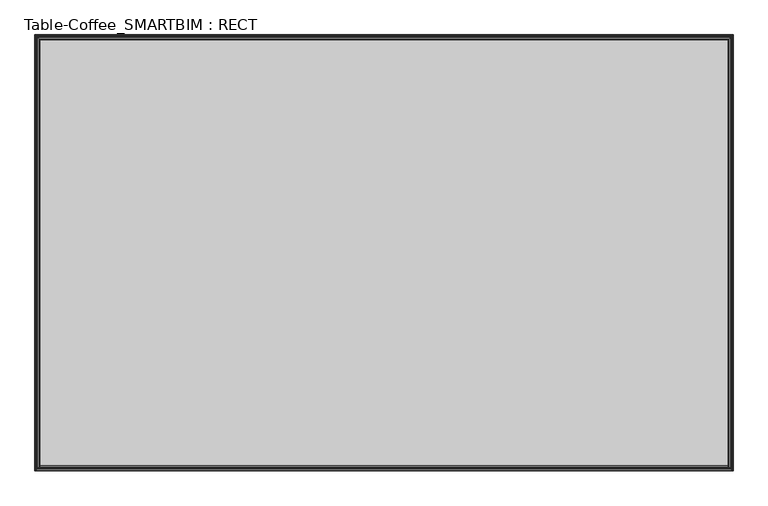
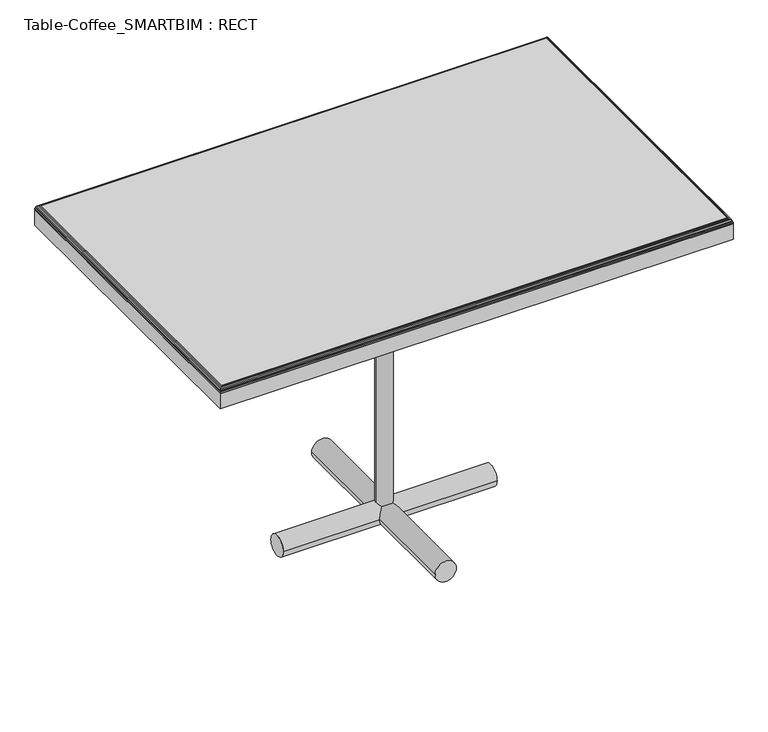
"""IFC4 building model written with IfcOpenShell, lengths in millimetres: furniture geometry, Table-Coffee_SMARTBIM : RECT."""

from ifc_helpers import new_model, si_unit, point, frame, frame_2d, origin, origin_2d, place, context, project, spatial, polyline, circle_curve, ellipse_curve, trimmed, segment, composite_curve, outline, extrude, source, transform, mapped, element, save
from ifc_brep_helpers import plane_surface, cylinder_surface, advanced_brep


def table_coffee_smartbim_rect_06f34b69(model_context):
    return source(origin(), model_context, "Body", "SolidModel", [
        extrude(outline(composite_curve([segment(trimmed(circle_curve(frame_2d((0.0, 25.4)), 25.4), [point((-25.4, 25.4))], [point((25.4, 25.4))], False, "CARTESIAN"), True, "CONTINUOUS"), segment(trimmed(circle_curve(frame_2d((0.0, 25.4)), 25.4), [point((25.4, 25.4))], [point((-25.4, 25.4))], False, "CARTESIAN"), True, "CONTINUOUS")], self_intersect=False)), frame((-254.0, 0.0, 0.0), z_axis=(1.0, 0.0, 0.0), x_axis=(0.0, 1.0, 0.0)), (0.0, 0.0, 1.0), 508.0),
        extrude(outline(composite_curve([segment(trimmed(circle_curve(frame_2d((25.4, 0.0)), 25.4), [point((25.4, -25.4))], [point((25.4, 25.4))], False, "CARTESIAN"), True, "CONTINUOUS"), segment(trimmed(circle_curve(frame_2d((25.4, 0.0)), 25.4), [point((25.4, 25.4))], [point((25.4, -25.4))], False, "CARTESIAN"), True, "CONTINUOUS")], self_intersect=False)), frame((0.0, -254.0, 0.0), z_axis=(0.0, 1.0, 0.0), x_axis=(0.0, 0.0, 1.0)), (0.0, 0.0, 1.0), 508.0),
        extrude(outline(polyline([(609.6, -381.0), (-609.6, -381.0), (-609.6, 381.0), (609.6, 381.0), (609.6, -381.0)])), frame((0.0, 0.0, 723.9), z_axis=(0.0, 0.0, 1.0), x_axis=(1.0, 0.0, 0.0)), (0.0, 0.0, 1.0), 38.1),
        advanced_brep(
        [(-600.1998654, 371.5998654, 774.7), (-600.1998654, -371.5998654, 774.7), (600.1998654, -371.5998654, 774.7), (600.1998654, 371.5998654, 774.7), (609.6, -381.0, 762.0), (-609.6, -381.0, 762.0), (-609.6, 381.0, 762.0), (609.6, 381.0, 762.0), (609.6, -381.0, 765.2998654), (-609.6, -381.0, 765.2998654), (-609.6, 381.0, 765.2998654), (609.6, 381.0, 765.2998654), (-609.2372483, -380.6372483, 767.8860287), (-609.2372483, 380.6372483, 767.8860287), (-602.3616212, -373.7616212, 774.4480533), (-602.3616212, 373.7616212, 774.4480533), (-604.3639185, 375.7639185, 773.7273912), (-604.3639185, -375.7639185, 773.7273912), (-606.4885738, 377.8885738, 772.2866155), (-606.4885738, -377.8885738, 772.2866155), (-608.5102962, 379.9102962, 769.692959), (-608.5102962, -379.9102962, 769.692959), (609.2372483, 380.6372483, 767.8860287), (602.3616212, 373.7616212, 774.4480533), (604.3639185, 375.7639185, 773.7273912), (606.4885738, 377.8885738, 772.2866155), (608.5102962, 379.9102962, 769.692959), (609.2372483, -380.6372483, 767.8860287), (602.3616212, -373.7616212, 774.4480533), (604.3639185, -375.7639185, 773.7273912), (606.4885738, -377.8885738, 772.2866155), (608.5102962, -379.9102962, 769.692959)],
        [
            (0, 1),
            (1, 2),
            (2, 3),
            (3, 0),
            (4, 5),
            (5, 6),
            (6, 7),
            (7, 4),
            (4, 8),
            (8, 9),
            (9, 5),
            (9, 10),
            (10, 6),
            (10, 11),
            (11, 7),
            (11, 8),
            (9, 12, ellipse_curve(frame((-600.1998654, -371.5998654, 765.2998654), z_axis=(-0.7071067811865475, 0.7071067811865475, 0.0), x_axis=(0.7071067811865474, 0.7071067811865476, 0.0)), 13.2937978, 9.4001346)),
            (12, 13),
            (13, 10, ellipse_curve(frame((-600.1998654, 371.5998654, 765.2998654), z_axis=(-0.7071067811865475, -0.7071067811865475, 0.0), x_axis=(-0.7071067811865474, 0.7071067811865476, 0.0)), 13.2937978, 9.4001346)),
            (14, 1, ellipse_curve(frame((-600.1998654, -371.5998654, 765.2998654), z_axis=(-0.7071067811865475, 0.7071067811865475, 0.0), x_axis=(0.7071067811865474, 0.7071067811865476, 0.0)), 13.2937978, 9.4001346)),
            (0, 15, ellipse_curve(frame((-600.1998654, 371.5998654, 765.2998654), z_axis=(-0.7071067811865475, -0.7071067811865475, 0.0), x_axis=(-0.7071067811865474, 0.7071067811865476, 0.0)), 13.2937978, 9.4001346)),
            (15, 14),
            (15, 16, ellipse_curve(frame((-600.1998654, 371.5998654, 765.2998654), z_axis=(-0.7071067811865475, -0.7071067811865475, 0.0), x_axis=(-0.7071067811865474, 0.7071067811865476, 0.0)), 13.2937978, 9.4001346)),
            (16, 17),
            (17, 14, ellipse_curve(frame((-600.1998654, -371.5998654, 765.2998654), z_axis=(-0.7071067811865475, 0.7071067811865475, 0.0), x_axis=(0.7071067811865474, 0.7071067811865476, 0.0)), 13.2937978, 9.4001346)),
            (16, 18, ellipse_curve(frame((-600.1998654, 371.5998654, 765.2998654), z_axis=(-0.7071067811865475, -0.7071067811865475, 0.0), x_axis=(-0.7071067811865474, 0.7071067811865476, 0.0)), 13.2937978, 9.4001346)),
            (18, 19),
            (19, 17, ellipse_curve(frame((-600.1998654, -371.5998654, 765.2998654), z_axis=(-0.7071067811865475, 0.7071067811865475, 0.0), x_axis=(0.7071067811865474, 0.7071067811865476, 0.0)), 13.2937978, 9.4001346)),
            (18, 20, ellipse_curve(frame((-600.1998654, 371.5998654, 765.2998654), z_axis=(-0.7071067811865475, -0.7071067811865475, 0.0), x_axis=(-0.7071067811865474, 0.7071067811865476, 0.0)), 13.2937978, 9.4001346)),
            (20, 21),
            (21, 19, ellipse_curve(frame((-600.1998654, -371.5998654, 765.2998654), z_axis=(-0.7071067811865475, 0.7071067811865475, 0.0), x_axis=(0.7071067811865474, 0.7071067811865476, 0.0)), 13.2937978, 9.4001346)),
            (12, 21, ellipse_curve(frame((-600.1998654, -371.5998654, 765.2998654), z_axis=(-0.7071067811865475, 0.7071067811865475, 0.0), x_axis=(0.7071067811865474, 0.7071067811865476, 0.0)), 13.2937978, 9.4001346)),
            (20, 13, ellipse_curve(frame((-600.1998654, 371.5998654, 765.2998654), z_axis=(-0.7071067811865475, -0.7071067811865475, 0.0), x_axis=(-0.7071067811865474, 0.7071067811865476, 0.0)), 13.2937978, 9.4001346)),
            (13, 22),
            (22, 11, ellipse_curve(frame((600.1998654, 371.5998654, 765.2998654), z_axis=(-0.7071067811865475, 0.7071067811865475, 0.0), x_axis=(0.7071067811865476, 0.7071067811865474, 0.0)), 13.2937978, 9.4001346)),
            (3, 23, ellipse_curve(frame((600.1998654, 371.5998654, 765.2998654), z_axis=(-0.7071067811865475, 0.7071067811865475, 0.0), x_axis=(0.7071067811865476, 0.7071067811865474, 0.0)), 13.2937978, 9.4001346)),
            (23, 15),
            (23, 24, ellipse_curve(frame((600.1998654, 371.5998654, 765.2998654), z_axis=(-0.7071067811865475, 0.7071067811865475, 0.0), x_axis=(0.7071067811865476, 0.7071067811865474, 0.0)), 13.2937978, 9.4001346)),
            (24, 16),
            (24, 25, ellipse_curve(frame((600.1998654, 371.5998654, 765.2998654), z_axis=(-0.7071067811865475, 0.7071067811865475, 0.0), x_axis=(0.7071067811865476, 0.7071067811865474, 0.0)), 13.2937978, 9.4001346)),
            (25, 18),
            (25, 26, ellipse_curve(frame((600.1998654, 371.5998654, 765.2998654), z_axis=(-0.7071067811865475, 0.7071067811865475, 0.0), x_axis=(0.7071067811865476, 0.7071067811865474, 0.0)), 13.2937978, 9.4001346)),
            (26, 20),
            (26, 22, ellipse_curve(frame((600.1998654, 371.5998654, 765.2998654), z_axis=(-0.7071067811865475, 0.7071067811865475, 0.0), x_axis=(0.7071067811865476, 0.7071067811865474, 0.0)), 13.2937978, 9.4001346)),
            (22, 27),
            (27, 8, ellipse_curve(frame((600.1998654, -371.5998654, 765.2998654), z_axis=(0.7071067811865475, 0.7071067811865475, 0.0), x_axis=(0.7071067811865474, -0.7071067811865476, 0.0)), 13.2937978, 9.4001346)),
            (2, 28, ellipse_curve(frame((600.1998654, -371.5998654, 765.2998654), z_axis=(0.7071067811865475, 0.7071067811865475, 0.0), x_axis=(0.7071067811865474, -0.7071067811865476, 0.0)), 13.2937978, 9.4001346)),
            (28, 23),
            (28, 29, ellipse_curve(frame((600.1998654, -371.5998654, 765.2998654), z_axis=(0.7071067811865475, 0.7071067811865475, 0.0), x_axis=(0.7071067811865474, -0.7071067811865476, 0.0)), 13.2937978, 9.4001346)),
            (29, 24),
            (29, 30, ellipse_curve(frame((600.1998654, -371.5998654, 765.2998654), z_axis=(0.7071067811865475, 0.7071067811865475, 0.0), x_axis=(0.7071067811865474, -0.7071067811865476, 0.0)), 13.2937978, 9.4001346)),
            (30, 25),
            (30, 31, ellipse_curve(frame((600.1998654, -371.5998654, 765.2998654), z_axis=(0.7071067811865475, 0.7071067811865475, 0.0), x_axis=(0.7071067811865474, -0.7071067811865476, 0.0)), 13.2937978, 9.4001346)),
            (31, 26),
            (31, 27, ellipse_curve(frame((600.1998654, -371.5998654, 765.2998654), z_axis=(0.7071067811865475, 0.7071067811865475, 0.0), x_axis=(0.7071067811865474, -0.7071067811865476, 0.0)), 13.2937978, 9.4001346)),
            (27, 12),
            (14, 28),
            (17, 29),
            (19, 30),
            (21, 31),
        ],
        [
            plane_surface(frame((-609.6, -381.0, 774.7), z_axis=(0.0, 0.0, 1.0), x_axis=(-1.0, 0.0, 0.0))),
            plane_surface(frame((-609.6, -381.0, 762.0), z_axis=(0.0, 0.0, -1.0), x_axis=(1.0, 0.0, 0.0))),
            plane_surface(frame((609.6, -381.0, 774.7), z_axis=(0.0, -1.0, 0.0), x_axis=(0.0, 0.0, -1.0))),
            plane_surface(frame((-609.6, -381.0, 774.7), z_axis=(-1.0, 0.0, 0.0), x_axis=(0.0, 0.0, -1.0))),
            plane_surface(frame((-609.6, 381.0, 774.7), z_axis=(0.0, 1.0, 0.0), x_axis=(0.0, 0.0, -1.0))),
            plane_surface(frame((609.6, 381.0, 774.7), z_axis=(1.0, 0.0, 0.0), x_axis=(0.0, 0.0, -1.0))),
            cylinder_surface(frame((-600.1998654, -381.0, 765.2998654), z_axis=(0.0, 1.0, 0.0), x_axis=(1.0, 0.0, 0.0)), 9.4001346),
            cylinder_surface(frame((-609.6, 371.5998654, 765.2998654), z_axis=(1.0, 0.0, 0.0), x_axis=(0.0, -1.0, 0.0)), 9.4001346),
            cylinder_surface(frame((600.1998654, 381.0, 765.2998654), z_axis=(0.0, -1.0, 0.0), x_axis=(-1.0, 0.0, 0.0)), 9.4001346),
            cylinder_surface(frame((609.6, -371.5998654, 765.2998654), z_axis=(-1.0, 0.0, 0.0), x_axis=(0.0, 1.0, 0.0)), 9.4001346),
        ],
        [
            (0, [[1, 2, 3, 4]]),
            (1, [[5, 6, 7, 8]]),
            (2, [[9, 10, 11, -5]]),
            (3, [[-11, 12, 13, -6]]),
            (4, [[-13, 14, 15, -7]]),
            (5, [[-15, 16, -9, -8]]),
            (6, [[-12, 17, 18, 19]]),
            (6, [[20, -1, 21, 22]]),
            (6, [[23, 24, 25, -22]]),
            (6, [[26, 27, 28, -24]]),
            (6, [[29, 30, 31, -27]]),
            (6, [[32, -30, 33, -18]]),
            (7, [[34, 35, -14, -19]]),
            (7, [[-4, 36, 37, -21]]),
            (7, [[-37, 38, 39, -23]]),
            (7, [[-39, 40, 41, -26]]),
            (7, [[-41, 42, 43, -29]]),
            (7, [[-43, 44, -34, -33]]),
            (8, [[45, 46, -16, -35]]),
            (8, [[-3, 47, 48, -36]]),
            (8, [[-48, 49, 50, -38]]),
            (8, [[-50, 51, 52, -40]]),
            (8, [[-52, 53, 54, -42]]),
            (8, [[-54, 55, -45, -44]]),
            (9, [[-10, -46, 56, -17]]),
            (9, [[57, -47, -2, -20]]),
            (9, [[58, -49, -57, -25]]),
            (9, [[59, -51, -58, -28]]),
            (9, [[60, -53, -59, -31]]),
            (9, [[-56, -55, -60, -32]]),
        ],
    ),
        extrude(outline(polyline([(76.2, -76.2), (-76.2, -76.2), (-76.2, 76.2), (76.2, 76.2), (76.2, -76.2)])), frame((0.0, 0.0, 755.65), z_axis=(0.0, 0.0, 1.0), x_axis=(1.0, 0.0, 0.0)), (0.0, 0.0, 1.0), 6.35),
        extrude(outline(composite_curve([segment(trimmed(circle_curve(origin_2d(), 19.05), [point((-19.05, 0.0))], [point((19.05, 0.0))], False, "CARTESIAN"), True, "CONTINUOUS"), segment(trimmed(circle_curve(origin_2d(), 19.05), [point((19.05, 0.0))], [point((-19.05, 0.0))], False, "CARTESIAN"), True, "CONTINUOUS")], self_intersect=False)), frame((0.0, 0.0, 24.2070278), z_axis=(0.0, 0.0, 1.0), x_axis=(1.0, 0.0, 0.0)), (0.0, 0.0, 1.0), 731.4429722),
    ])


if __name__ == "__main__":
    model = new_model("IFC4")
    model_context = context("Model", 3, world=origin())
    ifc_project = project(units=[si_unit("LENGTHUNIT", "METRE", prefix="MILLI")], contexts=[model_context])
    site = spatial("IfcSite", under=ifc_project)
    building = spatial("IfcBuilding", under=site)
    placement = place(None, origin())
    table_coffee_smartbim_rect_shape = table_coffee_smartbim_rect_06f34b69(model_context)
    element("IfcFurniture", 1, ObjectType="Table-Coffee_SMARTBIM : RECT", at=placement, inside=building, context=model_context, shape_type="MappedRepresentation", body=[
        mapped(table_coffee_smartbim_rect_shape, transform((0.0, 0.0, 0.0), x_axis=(1.0, 0.0, 0.0), y_axis=(0.0, 1.0, 0.0), z_axis=(0.0, 0.0, 1.0))),
    ])
    save(model, "model.ifc")

# Revit data of these elements
# Type "Table-Coffee_SMARTBIM : RECT"
#   Subcategory = "Table\r\n"
#   SmartBIM Object Created By = "SMARTBIM, LLC"
#   Manufacturer = "SMARTBIM"
#   Assembly Code = "E2020200"
#   95 CSI = "12500"
#   04 CSI = "12 50 00"
#   table cloth = 0' - 1 1/2"
#   Width = 4' - 0"
#   SmartBIM Object Version = 3
#   Height = 2' - 6"
#   Depth = 2' - 6"
#   Default Elevation = 4' - 0"
#   white cloth_parameter = WOOD-OAKFIRE
#   Table Unit = MET
#   Glide = none
#   Glass = none
# Element 1 (IfcFurniture, "Table-Coffee_SMARTBIM : RECT")
#   Materials on its faces: "WOOD-OAKFIRE", "MET"
# Materials
#   "WOOD-OAKFIRE": class "Wood", colour RGB 198 202 183, transparency 0, Description = "Generic wood", Cost = 0
#   "MET": class "Metal", colour RGB 189 187 185, transparency 0
